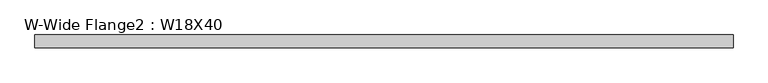
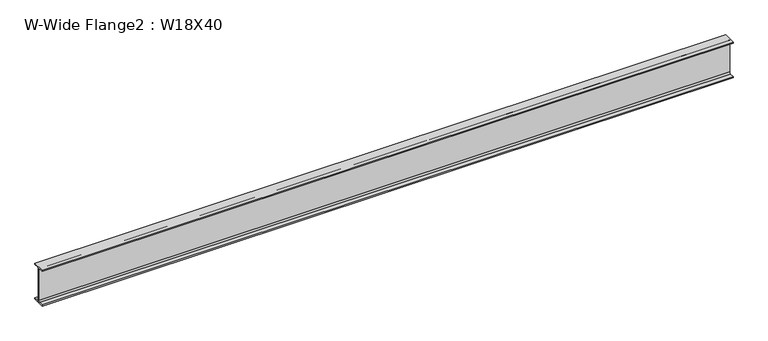
"""IFC4 building model written with IfcOpenShell, lengths in millimetres: beam geometry, W-Wide Flange2 : W18X40."""

from ifc_helpers import new_model, si_unit, point, frame, frame_2d, origin, place, context, project, spatial, polyline, circle_curve, trimmed, segment, composite_curve, outline, extrude, source, transform, mapped, element, save


def w_wide_flange2_w18x40_7e90f4d4(model_context):
    return source(origin(), model_context, "Body", "SweptSolid", [
        extrude(outline(composite_curve([segment(polyline([(76.454, -213.995), (76.454, -227.33), (-76.454, -227.33), (-76.454, -213.995), (-20.828, -213.995)]), True, "CONTINUOUS"), segment(trimmed(circle_curve(frame_2d((-20.828, -197.1675)), 16.8275), [point((-20.828, -213.995))], [point((-4.0005, -197.1675))], True, "CARTESIAN"), True, "CONTINUOUS"), segment(polyline([(-4.0005, -197.1675), (-4.0005, 197.1675)]), True, "CONTINUOUS"), segment(trimmed(circle_curve(frame_2d((-20.828, 197.1675)), 16.8275), [point((-4.0005, 197.1675))], [point((-20.828, 213.995))], True, "CARTESIAN"), True, "CONTINUOUS"), segment(polyline([(-20.828, 213.995), (-76.454, 213.995), (-76.454, 227.33), (76.454, 227.33), (76.454, 213.995), (20.828, 213.995)]), True, "CONTINUOUS"), segment(trimmed(circle_curve(frame_2d((20.828, 197.1675)), 16.8275), [point((20.828, 213.995))], [point((4.0005, 197.1675))], True, "CARTESIAN"), True, "CONTINUOUS"), segment(polyline([(4.0005, 197.1675), (4.0005, -197.1675)]), True, "CONTINUOUS"), segment(trimmed(circle_curve(frame_2d((20.828, -197.1675)), 16.8275), [point((4.0005, -197.1675))], [point((20.828, -213.995))], True, "CARTESIAN"), True, "CONTINUOUS"), segment(polyline([(20.828, -213.995), (76.454, -213.995)]), True, "CONTINUOUS")], self_intersect=False)), frame((-4178.046, 0.0, 0.0), z_axis=(1.0, 0.0, 0.0), x_axis=(0.0, 1.0, 0.0)), (0.0, 0.0, 1.0), 8356.092),
    ])


if __name__ == "__main__":
    model = new_model("IFC4")
    model_context = context("Model", 3, world=origin())
    ifc_project = project(units=[si_unit("LENGTHUNIT", "METRE", prefix="MILLI")], contexts=[model_context])
    site = spatial("IfcSite", under=ifc_project)
    building = spatial("IfcBuilding", under=site)
    placement = place(None, origin())
    w_wide_flange2_w18x40_shape = w_wide_flange2_w18x40_7e90f4d4(model_context)
    element("IfcBeam", 1, ObjectType="W-Wide Flange2 : W18X40", at=placement, inside=building, context=model_context, shape_type="MappedRepresentation", body=[
        mapped(w_wide_flange2_w18x40_shape, transform((0.0, 0.0, 0.0), x_axis=(1.0, 0.0, 0.0), y_axis=(0.0, 1.0, 0.0), z_axis=(0.0, 0.0, 1.0))),
    ])
    save(model, "model.ifc")

# Revit data of these elements
# Type "W-Wide Flange2 : W18X40"
#   Assembly Code = "B10"
#   W = 40
#   Length [instance default] = 5' - 0"
#   bf = 0' - 6.02"
#   d = 1' - 5.9"
#   k = 0' - 1 3/16"
#   k2 = 0' - 0.6625"
#   tf = 0' - 0.525"
#   tw = 0' - 0.315"
#   A = 0.0819444 SF
#   Structural Material [instance default] = Steel ASTM A992
# Element 1 (IfcBeam, "W-Wide Flange2 : W18X40")
#   Materials on its faces: "Steel ASTM A992"
# Materials
#   "Steel ASTM A992": class "Metal", colour RGB 199 199 199, transparency 0, Description = "Structural steel 50ksi", Cost = 0
